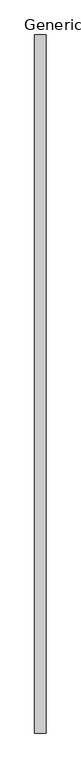
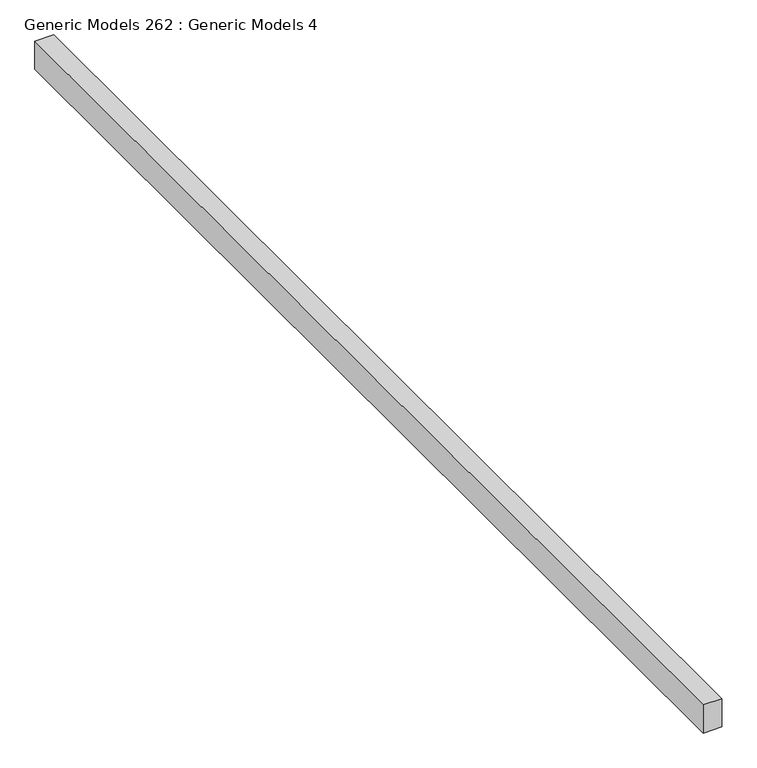
"""IFC4 building model written with IfcOpenShell, lengths in millimetres: proxy geometry, Generic Models 262 : Generic Models 4."""

from ifc_helpers import new_model, si_unit, frame, origin, place, context, project, spatial, polyline, outline, extrude, source, transform, mapped, element, save


def generic_models_262_generic_models_4_95232992(model_context):
    return source(origin(), model_context, "Body", "SweptSolid", [
        extrude(outline(polyline([(1625.4263704, -5493.3230338), (1422.2263704, -5493.3230338), (1422.2263704, 7054.2769662), (1625.4263704, 7054.2769662), (1625.4263704, -5493.3230338)])), frame((0.0, 0.0, 122908.8419635), z_axis=(0.0, 0.0, 1.0), x_axis=(1.0, 0.0, 0.0)), (0.0, 0.0, 1.0), 323.7665364),
    ])


if __name__ == "__main__":
    model = new_model("IFC4")
    model_context = context("Model", 3, world=origin())
    ifc_project = project(units=[si_unit("LENGTHUNIT", "METRE", prefix="MILLI")], contexts=[model_context])
    site = spatial("IfcSite", under=ifc_project)
    building = spatial("IfcBuilding", under=site)
    placement = place(None, origin())
    generic_models_262_generic_models_4_shape = generic_models_262_generic_models_4_95232992(model_context)
    element("IfcBuildingElementProxy", 1, Name="Generic Models 262 : Generic Models 4", ObjectType="Generic Models 262 : Generic Models 4", at=placement, inside=building, context=model_context, shape_type="MappedRepresentation", body=[
        mapped(generic_models_262_generic_models_4_shape, transform((0.0, 0.0, 0.0), x_axis=(1.0, 0.0, 0.0), y_axis=(0.0, 1.0, 0.0), z_axis=(0.0, 0.0, 1.0))),
    ])
    save(model, "model.ifc")

# Revit data of these elements
# Element 1 (IfcBuildingElementProxy, "Generic Models 262 : Generic Models 4")
#   Materials on its faces: "_ 8\" CONCRETE SLAB W/ GRADE BEAM (SEE STRUCT. DWGS)"
# Materials
#   "_ 8\" CONCRETE SLAB W/ GRADE BEAM (SEE STRUCT. DWGS)": class "Generic", colour RGB 191 191 191, transparency 0, Cost = 0
